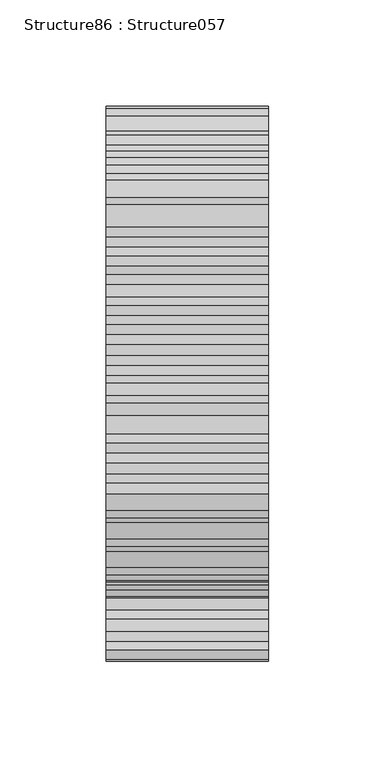
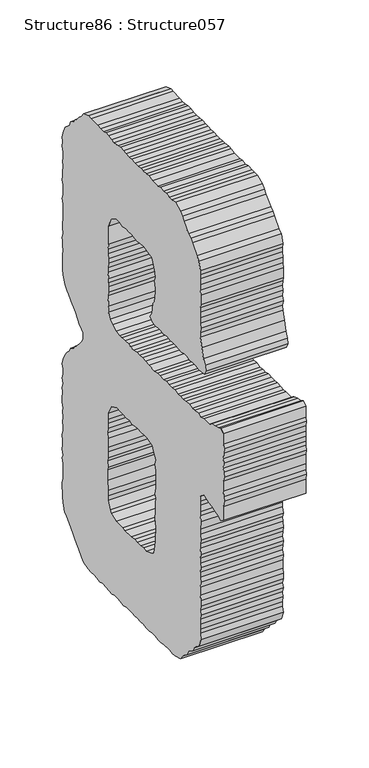
"""IFC4 building model written with IfcOpenShell, lengths in millimetres: proxy geometry, Structure86 : Structure057."""

from ifc_helpers import new_model, si_unit, frame, origin, place, context, project, spatial, polyline, outline, extrude, source, transform, mapped, element, save


def structure86_structure057_a961e1b5(model_context):
    return source(origin(), model_context, "Body", "SweptSolid", [
        extrude(outline(polyline([(275845.6324478, 3904.3901392), (275845.6324478, 3895.0048075), (275846.8134367, 3890.320967), (275845.6324478, 3885.0626781), (275845.6324478, 3870.9790644), (275846.2341745, 3866.8776953), (275846.2341745, 3861.6178018), (275845.6324478, 3856.9179152), (275846.8134367, 3852.2340747), (275846.2341745, 3849.3008577), (275846.2341745, 3843.432819), (275845.6324478, 3839.9331766), (275846.2341745, 3835.2332901), (275846.2341745, 3821.1737455), (275845.6324478, 3815.9154565), (275842.1119455, 3808.290376), (275838.6123031, 3804.7730829), (275836.2503253, 3802.448011), (275832.1714207, 3798.3305959), (275825.1288115, 3791.8865042), (275821.6083093, 3787.7867397), (275819.2687959, 3784.2614236), (275815.1674268, 3781.3282066), (275812.8279135, 3779.0031347), (275812.8279135, 3772.5606477), (275815.1674268, 3769.0176809), (275818.6670692, 3764.9435901), (275821.6083093, 3761.418274), (275826.2889406, 3757.8753073), (275828.6509184, 3753.8012165), (275833.3299451, 3751.4424479), (275835.6710631, 3747.3587295), (275839.1915653, 3743.8414364), (275842.1119455, 3739.7416719), (275845.6324478, 3733.2991849), (275846.8134367, 3728.0152223), (275845.6324478, 3723.9154578), (275845.6324478, 3719.2316172), (275846.8134367, 3714.5301261), (275845.6324478, 3709.2718371), (275846.8134367, 3705.1720727), (275846.2341745, 3700.4705815), (275846.8134367, 3694.6298211), (275846.8134367, 3690.512406), (275845.6324478, 3685.8285655), (275846.2341745, 3682.3289231), (275845.6324478, 3676.4432338), (275846.2341745, 3672.3691429), (275845.6324478, 3667.0851803), (275845.6324478, 3663.5598643), (275846.8134367, 3658.8840468), (275846.2341745, 3652.9999621), (275846.2341745, 3648.9258713), (275846.8134367, 3644.8245022), (275845.6324478, 3638.9580681), (275846.8134367, 3636.0408972), (275845.6324478, 3631.3410106), (275845.6324478, 3616.0972679), (275846.8134367, 3612.0135494), (275846.8134367, 3606.7295868), (275846.2341745, 3603.2122938), (275846.2341745, 3597.9540049), (275845.6324478, 3593.2541183), (275842.6912077, 3585.0706354), (275839.793292, 3582.7102621), (275835.0918009, 3578.0103756), (275832.7506829, 3575.6853037), (275828.6509184, 3570.9854171), (275826.2889406, 3568.0682461), (275821.6083093, 3564.54293), (275819.8480581, 3561.6257591), (275815.7466891, 3557.5003209), (275812.2261868, 3554.5831499), (275805.2060421, 3552.242032), (275800.5254108, 3551.6675836), (275794.6637906, 3552.242032), (275791.1432883, 3552.242032), (275785.8833948, 3551.0658569), (275781.7611658, 3552.242032), (275775.8995456, 3552.242032), (275766.5174231, 3551.0658569), (275762.4385185, 3552.242032), (275757.7578872, 3552.242032), (275753.6356582, 3551.6675836), (275747.7965025, 3551.0658569), (275743.6726689, 3552.242032), (275734.8922731, 3552.242032), (275729.6115197, 3551.6675836), (275726.1118773, 3552.242032), (275720.8519838, 3551.6675836), (275716.1504926, 3552.242032), (275712.0491235, 3551.0658569), (275706.1650388, 3551.0658569), (275701.4860121, 3552.242032), (275697.4071075, 3552.242032), (275692.7056163, 3551.0658569), (275688.024985, 3551.0658569), (275682.7650915, 3552.242032), (275674.5414934, 3552.242032), (275669.2591354, 3551.6675836), (275665.1818354, 3552.242032), (275656.9582374, 3554.0087015), (275653.458595, 3558.684519), (275651.1190816, 3561.025637), (275646.4159858, 3564.54293), (275644.0764725, 3569.2524442), (275641.1352324, 3571.5678885), (275636.4546011, 3574.5107332), (275634.1150878, 3578.6104977), (275630.0137187, 3582.7102621), (275626.4932164, 3585.0706354), (275623.5503718, 3593.2541183), (275624.7313607, 3598.5284533), (275624.7313607, 3602.6298224), (275624.1520985, 3607.8961343), (275624.7313607, 3612.5976255), (275623.5503718, 3617.2718384), (275624.7313607, 3621.3732075), (275623.5503718, 3626.0554434), (275623.5503718, 3631.3410106), (275624.1520985, 3636.0408972), (275624.1520985, 3644.2420307), (275623.5503718, 3649.5003197), (275624.7313607, 3653.6000842), (275624.1520985, 3658.8840468), (275623.5503718, 3663.5598643), (275624.7313607, 3667.0851803), (275624.1520985, 3672.3691429), (275623.5503718, 3676.4432338), (275624.1520985, 3682.3289231), (275624.7313607, 3686.4030139), (275623.5503718, 3690.512406), (275624.7313607, 3695.786741), (275624.7313607, 3700.4705815), (275623.5503718, 3708.6717151), (275624.1520985, 3713.9556777), (275624.1520985, 3718.0554422), (275624.7313607, 3723.9154578), (275624.1520985, 3728.5992983), (275624.1520985, 3733.2991849), (275618.8713451, 3737.9750024), (275610.6702115, 3735.0578314), (275605.9895802, 3734.47536), (275600.7296866, 3732.1149867), (275596.0281955, 3731.5325153), (275591.3475641, 3729.1737467), (275587.2461951, 3732.1149867), (275587.2461951, 3745.6000829), (275586.0876706, 3751.4424479), (275586.6444684, 3755.559863), (275587.2461951, 3760.818152), (275587.2461951, 3770.2018791), (275586.0876706, 3774.8857196), (275586.6444684, 3779.5872107), (275587.2461951, 3783.0868532), (275586.6444684, 3788.3611881), (275587.2461951, 3792.4705802), (275586.6444684, 3798.3305959), (275586.0876706, 3803.0064134), (275587.2461951, 3806.5317294), (275587.2461951, 3817.090027), (275591.3475641, 3820.015221), (275595.4473286, 3817.6741031), (275600.1504244, 3817.090027), (275605.9895802, 3815.3313805), (275610.0893447, 3812.3901405), (275618.8713451, 3812.3901405), (275623.5503718, 3811.2043377), (275627.6742053, 3812.3901405), (275632.9340989, 3812.3901405), (275637.0563278, 3811.7884138), (275642.3162213, 3812.3901405), (275647.5969747, 3812.3901405), (275652.2776061, 3811.2043377), (275656.3789751, 3811.7884138), (275660.5012041, 3811.2043377), (275665.7610976, 3812.3901405), (275670.4417289, 3811.7884138), (275675.1432201, 3811.7884138), (275679.2221248, 3812.3901405), (275683.9011515, 3811.2043377), (275689.7852361, 3811.7884138), (275693.8866052, 3811.7884138), (275697.9863697, 3811.2043377), (275707.3476324, 3811.2043377), (275712.6283857, 3811.7884138), (275717.3090171, 3812.3901405), (275722.5913751, 3811.7884138), (275726.1118773, 3812.3901405), (275731.9734975, 3811.2043377), (275736.6525243, 3811.7884138), (275740.1746311, 3812.3901405), (275746.0362513, 3811.7884138), (275750.1360158, 3812.3901405), (275754.8166471, 3811.2043377), (275760.0765407, 3812.3901405), (275765.9590208, 3815.3313805), (275770.0603899, 3818.2309008), (275771.820641, 3824.1149855), (275771.820641, 3829.9733965), (275772.9791654, 3839.3587282), (275772.3999032, 3843.432819), (275772.3999032, 3848.7167816), (275771.820641, 3852.8181507), (275771.820641, 3856.9179152), (275772.9791654, 3862.8036045), (275772.9791654, 3866.8776953), (275772.3999032, 3871.5599312), (275772.3999032, 3876.263027), (275772.9791654, 3880.9452629), (275772.9791654, 3885.0626781), (275771.820641, 3890.905043), (275771.820641, 3908.46423), (275768.3001387, 3917.8479571), (275759.4972785, 3922.5494483), (275754.8166471, 3922.5494483), (275749.5567536, 3921.3748778), (275744.2535358, 3922.5494483), (275740.1746311, 3921.9733953), (275735.4939998, 3922.5494483), (275729.6115197, 3921.9733953), (275726.1118773, 3921.3748778), (275720.8519838, 3921.9733953), (275715.5487659, 3922.5494483), (275711.4698613, 3921.3748778), (275702.667001, 3919.6066036), (275700.3274877, 3916.6653636), (275697.4071075, 3908.46423), (275696.8053808, 3903.2059411), (275697.9863697, 3899.7046941), (275696.8053808, 3893.246161), (275696.8053808, 3889.1463965), (275697.9863697, 3879.1769888), (275700.9067499, 3875.686974), (275702.667001, 3865.1190488), (275705.6082411, 3860.4432313), (275701.4860121, 3856.9179152), (275696.8053808, 3855.7353217), (275692.1247495, 3856.9179152), (275688.024985, 3856.9179152), (275683.9011515, 3855.7353217), (275678.6428625, 3856.9179152), (275673.382969, 3856.3161885), (275668.6798732, 3856.9179152), (275664.5801087, 3856.9179152), (275655.1979862, 3855.7353217), (275650.5173549, 3856.9179152), (275646.4159858, 3856.9179152), (275641.1352324, 3855.7353217), (275637.0563278, 3856.9179152), (275632.353232, 3856.9179152), (275627.0949431, 3855.7353217), (275621.8125851, 3856.3161885), (275618.2920828, 3856.3161885), (275615.9734293, 3861.0192843), (275616.5302271, 3866.3032469), (275619.4730717, 3870.9790644), (275621.8125851, 3880.3627915), (275624.1520985, 3889.1463965), (275624.7313607, 3893.246161), (275623.5503718, 3898.5301236), (275624.7313607, 3902.6314927), (275624.1520985, 3908.46423), (275624.7313607, 3913.1641166), (275624.1520985, 3917.8479571), (275623.5503718, 3921.3748778), (275623.5503718, 3930.7329312), (275624.1520985, 3935.4328178), (275624.1520985, 3940.718385), (275624.7313607, 3945.9766739), (275624.7313607, 3950.0940891), (275624.1520985, 3954.1778075), (275626.4932164, 3962.3757319), (275630.0137187, 3965.3201811), (275637.63559, 3973.5197101), (275639.9751034, 3976.4368811), (275643.4972103, 3978.8036727), (275651.1190816, 3986.4046842), (275653.458595, 3989.9460463), (275656.9582374, 3992.8375436), (275664.5801087, 3996.9645864), (275669.8608621, 3996.390138), (275673.9622312, 3996.390138), (275679.2221248, 3996.9645864), (275683.9011515, 3995.7803883), (275688.6042472, 3996.9645864), (275692.7056163, 3995.7803883), (275701.4860121, 3995.7803883), (275707.3476324, 3996.9645864), (275710.8681346, 3996.9645864), (275716.7297548, 3996.390138), (275720.2502571, 3996.390138), (275724.9308884, 3995.7803883), (275729.6115197, 3995.7803883), (275734.8922731, 3996.390138), (275739.5729044, 3995.7803883), (275744.2535358, 3996.390138), (275748.3757647, 3996.390138), (275753.056396, 3996.9645864), (275757.178625, 3996.390138), (275763.0177807, 3995.7803883), (275767.698412, 3995.7803883), (275771.820641, 3996.9645864), (275776.5012723, 3996.9645864), (275780.6010368, 3995.7803883), (275785.2816681, 3995.7803883), (275789.9622994, 3996.390138), (275800.5254108, 3996.390138), (275804.0250532, 3996.9645864), (275812.2261868, 3994.0233463), (275815.1674268, 3989.9460463), (275819.2687959, 3986.4046842), (275822.7892982, 3982.3225704), (275825.7305382, 3979.9621971), (275828.6509184, 3976.4368811), (275833.3299451, 3973.5197101), (275835.0918009, 3968.8198235), (275842.1119455, 3962.9774586), (275845.6324478, 3955.360401), (275846.8134367, 3950.6765605), (275846.2341745, 3945.9766739), (275846.8134367, 3941.2912288), (275845.6324478, 3936.0345445), (275845.6324478, 3930.7329312), (275846.2341745, 3927.2332888), (275845.6324478, 3921.9733953), (275846.2341745, 3917.8479571), (275846.2341745, 3912.5896682), (275846.8134367, 3908.46423), (275845.6324478, 3904.3901392)]), holes=[polyline([(275702.667001, 3735.0578314), (275700.3274877, 3731.5325153), (275696.8053808, 3725.0996559), (275697.9863697, 3719.8140887), (275696.8053808, 3714.5301261), (275696.8053808, 3696.9709391), (275697.9863697, 3691.0868544), (275696.8053808, 3687.587212), (275697.4071075, 3681.7271964), (275697.4071075, 3672.9435914), (275697.9863697, 3667.6853024), (275697.4071075, 3662.9854159), (275696.8053808, 3659.4584952), (275696.8053808, 3654.7842823), (275697.4071075, 3650.1004418), (275697.4071075, 3644.8245022), (275697.9863697, 3640.114988), (275699.725761, 3631.915459), (275702.667001, 3629.5984101), (275710.8681346, 3626.6571701), (275715.5487659, 3627.2396415), (275719.6709949, 3626.6571701), (275725.5326151, 3626.6571701), (275729.6115197, 3627.2396415), (275735.4939998, 3626.0554434), (275745.4345247, 3626.0554434), (275748.9550269, 3626.6571701), (275759.4972785, 3626.6571701), (275767.1191498, 3630.1824862), (275768.8794009, 3632.5155811), (275772.3999032, 3639.5405396), (275771.820641, 3644.2420307), (275771.820641, 3649.5003197), (275772.9791654, 3658.8840468), (275772.9791654, 3668.8261762), (275771.820641, 3672.3691429), (275772.9791654, 3677.6274319), (275771.820641, 3681.7271964), (275772.3999032, 3687.0127636), (275771.820641, 3691.6869765), (275771.820641, 3700.4705815), (275772.9791654, 3705.1720727), (275771.820641, 3710.4560353), (275772.3999032, 3715.1302482), (275771.820641, 3719.2316172), (275771.820641, 3725.0996559), (275767.698412, 3733.8736333), (275759.4972785, 3737.9750024), (275753.6356582, 3737.400554), (275750.1360158, 3737.9750024), (275744.2535358, 3736.7988273), (275739.5729044, 3737.9750024), (275734.8922731, 3736.7988273), (275730.7925086, 3737.400554), (275725.5326151, 3737.9750024), (275719.6709949, 3737.400554), (275716.1504926, 3737.9750024), (275710.8681346, 3737.9750024), (275702.667001, 3735.0578314)])]), frame((-59031.6926606, 0.0, 0.0), z_axis=(1.0, 0.0, 0.0), x_axis=(0.0, 1.0, 0.0)), (0.0, 0.0, 1.0), 76.2),
    ])


if __name__ == "__main__":
    model = new_model("IFC4")
    model_context = context("Model", 3, world=origin())
    ifc_project = project(units=[si_unit("LENGTHUNIT", "METRE", prefix="MILLI")], contexts=[model_context])
    site = spatial("IfcSite", under=ifc_project)
    building = spatial("IfcBuilding", under=site)
    placement = place(None, origin())
    structure86_structure057_shape = structure86_structure057_a961e1b5(model_context)
    element("IfcBuildingElementProxy", 1, Name="Structure86 : Structure057", ObjectType="Structure86 : Structure057", at=placement, inside=building, context=model_context, shape_type="MappedRepresentation", body=[
        mapped(structure86_structure057_shape, transform((0.0, 0.0, 0.0), x_axis=(1.0, 0.0, 0.0), y_axis=(0.0, 1.0, 0.0), z_axis=(0.0, 0.0, 1.0))),
    ])
    save(model, "model.ifc")

# Revit data of these elements
# Type "Structure86 : Structure057"
#   NameOverride = "Structure057"
# Element 1 (IfcBuildingElementProxy, "Structure86 : Structure057")
#   Materials on its faces: "BRUSHED ALUM. LETTERING"
# Materials
#   "BRUSHED ALUM. LETTERING": class "Unassigned", colour RGB 169 181 186, transparency 0, Cost = 0
